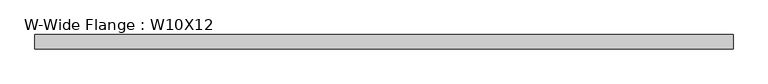
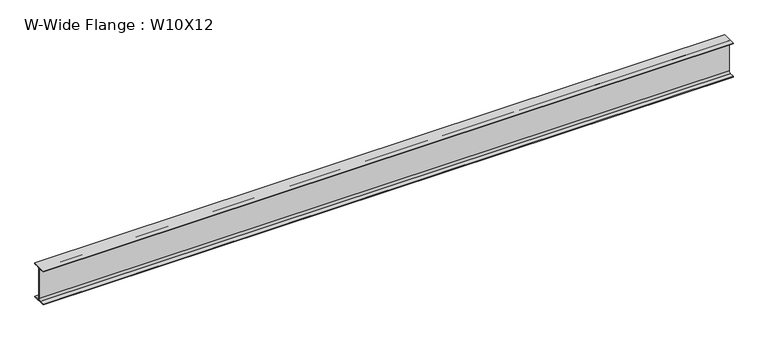
"""IFC4 building model written with IfcOpenShell, lengths in millimetres: beam geometry, W-Wide Flange : W10X12."""

import ifcopenshell
import ifcopenshell.guid

model = None  # the IFC model being written
_history = None  # IfcOwnerHistory: only IFC2X3 demands one
_inside = {}  # id of a spatial element -> (the spatial element, [elements in it])
_under = {}  # id of a project, library or spatial element -> (it, [spatial elements below it])
_declared = {}  # id of a project -> (the project, [libraries it declares])
_typed = {}  # id of a type object -> (the type object, [elements of that type])
_made_of = {}  # id of a material, layer set ... -> (it, [elements and type objects made of it])


def new_model(schema):
    """Start an empty IFC model of exactly this schema.

    Asked for "IFC4X3", IfcOpenShell would pick the latest addendum, in which some entities
    have other attributes; the version numbers below select the first issue.
    IFC2X3 requires an IfcOwnerHistory on every rooted entity: one is made here for all.
    """
    global model, _history
    if schema == "IFC4X3":
        model = ifcopenshell.file(schema_version=(4, 3, 0, 0))
    else:
        model = ifcopenshell.file(schema=schema)
    _inside.clear()
    _under.clear()
    _declared.clear()
    _typed.clear()
    _made_of.clear()
    _history = None
    if model.schema == "IFC2X3":
        org = make("IfcOrganization", Name="unknown")
        user = make(
            "IfcPersonAndOrganization",
            ThePerson=make("IfcPerson", FamilyName="unknown"),
            TheOrganization=org,
        )
        app = make(
            "IfcApplication",
            ApplicationDeveloper=org,
            Version="unknown",
            ApplicationFullName="unknown",
            ApplicationIdentifier="unknown",
        )
        _history = make(
            "IfcOwnerHistory",
            OwningUser=user,
            OwningApplication=app,
            ChangeAction="ADDED",
            CreationDate=0,
        )
    return model


def make(cls, **values):
    """One entity of the class cls with the attributes given. An attribute that is None is left unset."""
    return model.create_entity(
        cls, **{name: value for name, value in values.items() if value is not None}
    )


def rooted(cls, **values):
    """An entity with a GlobalId (a new one), such as an element, a storey or a relation."""
    return make(cls, GlobalId=ifcopenshell.guid.new(), OwnerHistory=_history, **values)


def si_unit(unit_type, name, prefix=None):
    """IfcSIUnit, for example si_unit("LENGTHUNIT", "METRE", prefix="MILLI")."""
    return make("IfcSIUnit", UnitType=unit_type, Prefix=prefix, Name=name)


def assignment(units):
    """IfcUnitAssignment: the units of a project."""
    return None if units is None else make("IfcUnitAssignment", Units=units)


def point(xyz):
    """IfcCartesianPoint."""
    return None if xyz is None else make("IfcCartesianPoint", Coordinates=xyz)


def direction(xyz):
    """IfcDirection."""
    return None if xyz is None else make("IfcDirection", DirectionRatios=xyz)


def frame(location, z_axis=None, x_axis=None):
    """IfcAxis2Placement3D, a coordinate frame: its origin and axes. An axis left out is left unset."""
    return make(
        "IfcAxis2Placement3D",
        Location=point(location),
        Axis=direction(z_axis),
        RefDirection=direction(x_axis),
    )


def frame_2d(location, x_axis=None):
    """IfcAxis2Placement2D, a coordinate frame in the plane: its origin and x axis."""
    return make(
        "IfcAxis2Placement2D", Location=point(location), RefDirection=direction(x_axis)
    )


def origin():
    """The frame at (0, 0, 0) with its axes left unset."""
    return frame((0.0, 0.0, 0.0))


def place(relative_to, where):
    """IfcLocalPlacement: puts the frame where relative to a parent placement (None: the world)."""
    return make(
        "IfcLocalPlacement", PlacementRelTo=relative_to, RelativePlacement=where
    )


def context(
    kind, dimensions, precision=None, world=None, true_north=None, identifier=None
):
    """IfcGeometricRepresentationContext, for example the 3D "Model" context."""
    return make(
        "IfcGeometricRepresentationContext",
        ContextIdentifier=identifier,
        ContextType=kind,
        CoordinateSpaceDimension=dimensions,
        Precision=precision,
        WorldCoordinateSystem=world,
        TrueNorth=true_north,
    )


def project(units=None, contexts=None):
    """IfcProject with its units and contexts."""
    return rooted(
        "IfcProject",
        Name="project",
        RepresentationContexts=contexts,
        UnitsInContext=assignment(units),
    )


def spatial(cls, under=None, at=None, **own):
    """A site, building, storey or space (cls), placed at a placement, below another one or the project."""
    s = rooted(cls, ObjectPlacement=at, **own)
    if under is not None:
        _under.setdefault(under.id(), (under, []))[1].append(s)
    return s


def polyline(points):
    """IfcPolyline through the points."""
    return make("IfcPolyline", Points=[point(p) for p in points])


def circle_curve(where, radius):
    """IfcCircle in the frame where."""
    return make("IfcCircle", Position=where, Radius=radius)


def trimmed(basis, trim1, trim2, sense, master):
    """IfcTrimmedCurve: the piece of a basis curve between two trims."""
    return make(
        "IfcTrimmedCurve",
        BasisCurve=basis,
        Trim1=trim1,
        Trim2=trim2,
        SenseAgreement=sense,
        MasterRepresentation=master,
    )


def segment(curve, same_sense, transition):
    """IfcCompositeCurveSegment."""
    return make(
        "IfcCompositeCurveSegment",
        Transition=transition,
        SameSense=same_sense,
        ParentCurve=curve,
    )


def composite_curve(segments, self_intersect=None):
    """IfcCompositeCurve: segments joined end to end."""
    return make("IfcCompositeCurve", Segments=segments, SelfIntersect=self_intersect)


def outline(outer, holes=None, kind="AREA"):
    """IfcArbitraryClosedProfileDef: a profile drawn as a closed curve; with holes, ...WithVoids."""
    if holes is None:
        return make("IfcArbitraryClosedProfileDef", ProfileType=kind, OuterCurve=outer)
    return make(
        "IfcArbitraryProfileDefWithVoids",
        ProfileType=kind,
        OuterCurve=outer,
        InnerCurves=holes,
    )


def extrude(swept, where, along, depth):
    """IfcExtrudedAreaSolid: the profile swept, set in the frame where, extruded along a direction by depth."""
    return make(
        "IfcExtrudedAreaSolid",
        SweptArea=swept,
        Position=where,
        ExtrudedDirection=direction(along),
        Depth=depth,
    )


def shape(context_of_items, identifier, shape_type, items):
    """IfcShapeRepresentation: the items that make up one representation, for example the "Body"."""
    return make(
        "IfcShapeRepresentation",
        ContextOfItems=context_of_items,
        RepresentationIdentifier=identifier,
        RepresentationType=shape_type,
        Items=items,
    )


def source(mapping_origin, context_of_items, identifier, shape_type, items):
    """IfcRepresentationMap: a shape defined once, which mapped items show again and again."""
    return make(
        "IfcRepresentationMap",
        MappingOrigin=mapping_origin,
        MappedRepresentation=shape(context_of_items, identifier, shape_type, items),
    )


def transform(
    local_origin,
    x_axis=None,
    y_axis=None,
    z_axis=None,
    scale=None,
    scale2=None,
    scale3=None,
    uniform=True,
):
    """IfcCartesianTransformationOperator3D, or its non-uniform kind. x_axis, y_axis, z_axis: its Axis1, 2, 3."""
    if uniform:
        return make(
            "IfcCartesianTransformationOperator3D",
            Axis1=direction(x_axis),
            Axis2=direction(y_axis),
            LocalOrigin=point(local_origin),
            Scale=scale,
            Axis3=direction(z_axis),
        )
    return make(
        "IfcCartesianTransformationOperator3DnonUniform",
        Axis1=direction(x_axis),
        Axis2=direction(y_axis),
        LocalOrigin=point(local_origin),
        Scale=scale,
        Axis3=direction(z_axis),
        Scale2=scale2,
        Scale3=scale3,
    )


def mapped(mapping_source, mapping_target):
    """IfcMappedItem: shows the shape of a source again, moved by a transform."""
    return make(
        "IfcMappedItem", MappingSource=mapping_source, MappingTarget=mapping_target
    )


def made_of(thing, what):
    """Note that an element or type object is made of a material, layer set ...; save() writes the relation."""
    if what is not None:
        _made_of.setdefault(what.id(), (what, []))[1].append(thing)
    return thing


def element(
    cls,
    number,
    at=None,
    inside=None,
    cuts=None,
    type_object=None,
    material=None,
    context=None,
    identifier="Body",
    shape_type=None,
    held_by="IfcProductDefinitionShape",
    body=None,
    shapes=None,
    **own,
):
    """One element of the class cls, such as IfcWall. Its Tag is "e" and its number.

    at: its placement. inside: the storey or other place that contains it. cuts: it is an
    opening in that element (IfcRelVoidsElement). A single representation is given by context,
    identifier, shape_type and body (its items); several are given by shapes. held_by: the class
    of the entity that holds the representations. save() writes the other relations.
    """
    e = rooted(cls, Tag="e%d" % number, ObjectPlacement=at, **own)
    if body is not None:
        shapes = [shape(context, identifier, shape_type, body)]
    if shapes is not None:
        e.Representation = make(held_by, Representations=shapes)
    if inside is not None:
        _inside.setdefault(inside.id(), (inside, []))[1].append(e)
    if cuts is not None:
        rooted(
            "IfcRelVoidsElement", RelatingBuildingElement=cuts, RelatedOpeningElement=e
        )
    if type_object is not None:
        _typed.setdefault(type_object.id(), (type_object, []))[1].append(e)
    return made_of(e, material)


def aggregate(whole, parts):
    """IfcRelAggregates: a whole, such as a stair, and the parts it consists of."""
    return rooted("IfcRelAggregates", RelatingObject=whole, RelatedObjects=parts)


def save(model, path):
    """Write the relations noted so far, then the file.

    IfcRelAggregates (storeys below a building ...), IfcRelContainedInSpatialStructure (elements
    in a storey), IfcRelDefinesByType, IfcRelAssociatesMaterial and IfcRelDeclares: one each for
    every whole, place, type object, material and project.
    """
    for whole, parts in _under.values():
        aggregate(whole, parts)
    for where, things in _inside.values():
        rooted(
            "IfcRelContainedInSpatialStructure",
            RelatedElements=things,
            RelatingStructure=where,
        )
    for kind, things in _typed.values():
        rooted("IfcRelDefinesByType", RelatedObjects=things, RelatingType=kind)
    for what, things in _made_of.values():
        rooted("IfcRelAssociatesMaterial", RelatedObjects=things, RelatingMaterial=what)
    for by, libraries in _declared.values():
        rooted("IfcRelDeclares", RelatingContext=by, RelatedDefinitions=libraries)
    model.write(path)


def w_wide_flange_w10x12_1bd4f99f(model_context):
    return source(origin(), model_context, "Body", "SweptSolid", [
        extrude(outline(composite_curve([segment(polyline([(50.292, -120.015), (50.292, -125.349), (-50.292, -125.349), (-50.292, -120.015), (-16.129, -120.015)]), True, "CONTINUOUS"), segment(trimmed(circle_curve(frame_2d((-16.129, -106.299)), 13.716), [point((-16.129, -120.015))], [point((-2.413, -106.299))], True, "CARTESIAN"), True, "CONTINUOUS"), segment(polyline([(-2.413, -106.299), (-2.413, 106.299)]), True, "CONTINUOUS"), segment(trimmed(circle_curve(frame_2d((-16.129, 106.299)), 13.716), [point((-2.413, 106.299))], [point((-16.129, 120.015))], True, "CARTESIAN"), True, "CONTINUOUS"), segment(polyline([(-16.129, 120.015), (-50.292, 120.015), (-50.292, 125.349), (50.292, 125.349), (50.292, 120.015), (16.129, 120.015)]), True, "CONTINUOUS"), segment(trimmed(circle_curve(frame_2d((16.129, 106.299)), 13.716), [point((16.129, 120.015))], [point((2.413, 106.299))], True, "CARTESIAN"), True, "CONTINUOUS"), segment(polyline([(2.413, 106.299), (2.413, -106.299)]), True, "CONTINUOUS"), segment(trimmed(circle_curve(frame_2d((16.129, -106.299)), 13.716), [point((2.413, -106.299))], [point((16.129, -120.015))], True, "CARTESIAN"), True, "CONTINUOUS"), segment(polyline([(16.129, -120.015), (50.292, -120.015)]), True, "CONTINUOUS")], self_intersect=False)), frame((-2408.2375, 0.0, 0.0), z_axis=(1.0, 0.0, 0.0), x_axis=(0.0, 1.0, 0.0)), (0.0, 0.0, 1.0), 4828.794),
    ])


if __name__ == "__main__":
    model = new_model("IFC4")
    model_context = context("Model", 3, world=origin())
    ifc_project = project(units=[si_unit("LENGTHUNIT", "METRE", prefix="MILLI")], contexts=[model_context])
    site = spatial("IfcSite", under=ifc_project)
    building = spatial("IfcBuilding", under=site)
    placement = place(None, origin())
    w_wide_flange_w10x12_shape = w_wide_flange_w10x12_1bd4f99f(model_context)
    element("IfcBeam", 1, ObjectType="W-Wide Flange : W10X12", at=placement, inside=building, context=model_context, shape_type="MappedRepresentation", body=[
        mapped(w_wide_flange_w10x12_shape, transform((0.0, 0.0, 0.0), x_axis=(1.0, 0.0, 0.0), y_axis=(0.0, 1.0, 0.0), z_axis=(0.0, 0.0, 1.0))),
    ])
    save(model, "model.ifc")

# Revit data of these elements
# Type "W-Wide Flange : W10X12"
#   Assembly Code = "B10"
#   W = 12
#   Length [instance default] = 1524 mm
#   bf = 100.584 mm
#   d = 250.698 mm
#   k = 19.05 mm
#   k2 = 13.716 mm
#   tf = 5.334 mm
#   tw = 4.826 mm
#   A = 0.00228387 m²
#   Structural Material [instance default] = Steel ASTM A992
# Element 1 (IfcBeam, "W-Wide Flange : W10X12")
#   Structural Material = Aluminum, Anodized Red
#   Materials on its faces: "Aluminum, Anodized Red"
# Materials
#   "Steel ASTM A992": class "Metal", colour RGB 128 0 0, transparency 0, Description = "Structural steel 50ksi", Cost = 0
#   "Aluminum, Anodized Red": class "Metal", colour RGB 120 120 120, transparency 0, Description = "Anodized aluminum, red", Cost = 0
